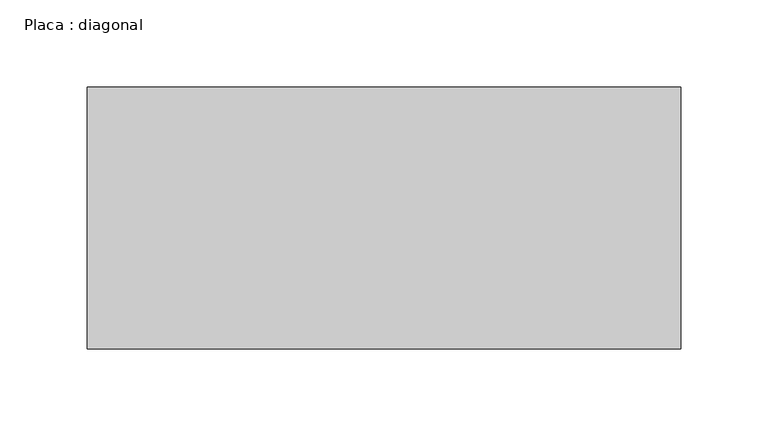
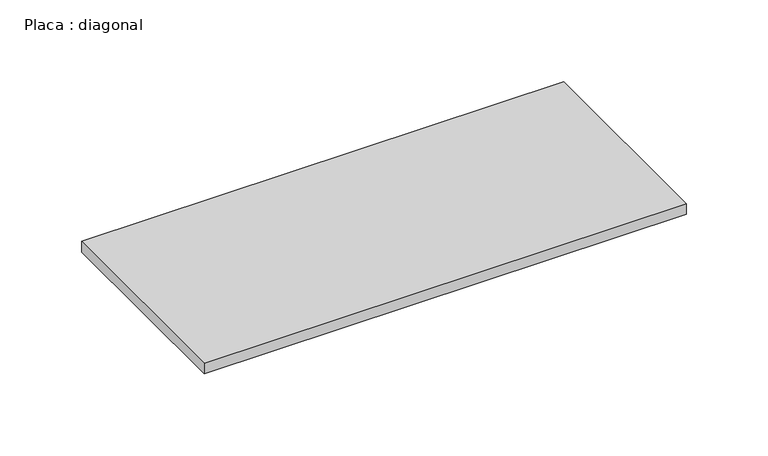
"""IFC4 building model written with IfcOpenShell, lengths in millimetres: beam geometry, Placa : diagonal."""

from ifc_helpers import new_model, si_unit, frame, origin, place, context, project, spatial, polyline, outline, extrude, source, transform, mapped, element, save


def placa_diagonal_348c000d(model_context):
    return source(origin(), model_context, "Body", "SweptSolid", [
        extrude(outline(polyline([(169.5917652, 75.0), (169.5917652, -75.0), (-170.4649339, -75.0), (-170.4649339, 75.0), (169.5917652, 75.0)])), frame((0.0, 0.0, -4.0), z_axis=(0.0, 0.0, 1.0), x_axis=(1.0, 0.0, 0.0)), (0.0, 0.0, 1.0), 8.0),
    ])


if __name__ == "__main__":
    model = new_model("IFC4")
    model_context = context("Model", 3, world=origin())
    ifc_project = project(units=[si_unit("LENGTHUNIT", "METRE", prefix="MILLI")], contexts=[model_context])
    site = spatial("IfcSite", under=ifc_project)
    building = spatial("IfcBuilding", under=site)
    placement = place(None, origin())
    placa_diagonal_shape = placa_diagonal_348c000d(model_context)
    element("IfcBeam", 1, ObjectType="Placa : diagonal", at=placement, inside=building, context=model_context, shape_type="MappedRepresentation", body=[
        mapped(placa_diagonal_shape, transform((0.0, 0.0, 0.0), x_axis=(1.0, 0.0, 0.0), y_axis=(0.0, 1.0, 0.0), z_axis=(0.0, 0.0, 1.0))),
    ])
    save(model, "model.ifc")

# Revit data of these elements
# Type "Placa : diagonal"
#   W = 0
#   Length [instance default] = 1.50 m
#   b = 0.15 m
#   d = 0.008 m
#   A = 0 m²
#   Structural Material [instance default] = Aço, 45-345
# Element 1 (IfcBeam, "Placa : diagonal")
#   Materials on its faces: "Aço, 45-345"
# Materials
#   "Aço, 45-345": class "Metal", colour RGB 247 247 247, transparency 0, Description = "Aço 345 MPa", Cost = 0
